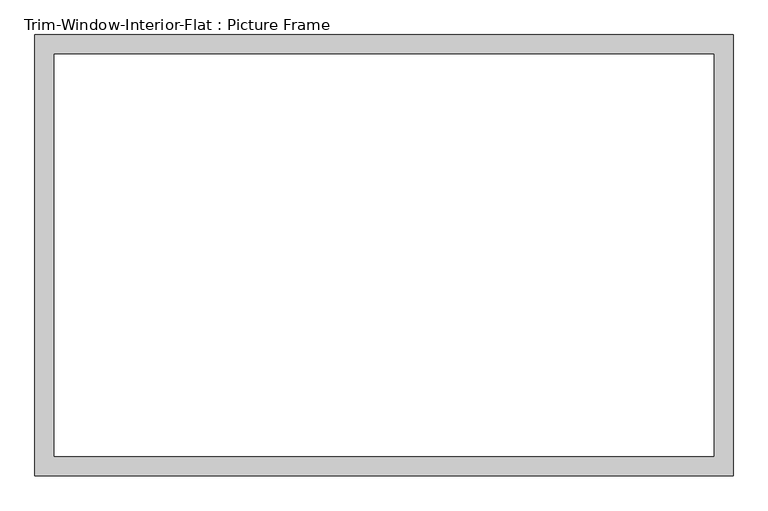
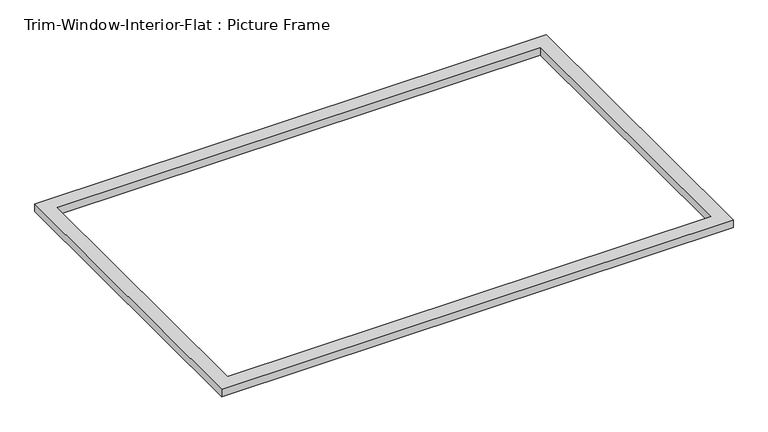
"""IFC4 building model written with IfcOpenShell, lengths in millimetres: proxy geometry, Trim-Window-Interior-Flat : Picture Frame."""

from ifc_helpers import new_model, si_unit, origin, origin_with_axes, place, context, project, spatial, polyline, outline, extrude, source, transform, mapped, element, save


def trim_window_interior_flat_picture_frame_b9d4c0b4(model_context):
    return source(origin(), model_context, "Body", "SweptSolid", [
        extrude(outline(polyline([(1035.05, 44.45), (1035.05, -1263.65), (-1035.05, -1263.65), (-1035.05, 44.45), (1035.05, 44.45)]), holes=[polyline([(977.9, -12.7), (-977.9, -12.7), (-977.9, -1206.5), (977.9, -1206.5), (977.9, -12.7)])]), origin_with_axes(), (0.0, 0.0, 1.0), 31.75),
    ])


if __name__ == "__main__":
    model = new_model("IFC4")
    model_context = context("Model", 3, world=origin())
    ifc_project = project(units=[si_unit("LENGTHUNIT", "METRE", prefix="MILLI")], contexts=[model_context])
    site = spatial("IfcSite", under=ifc_project)
    building = spatial("IfcBuilding", under=site)
    placement = place(None, origin())
    trim_window_interior_flat_picture_frame_shape = trim_window_interior_flat_picture_frame_b9d4c0b4(model_context)
    element("IfcBuildingElementProxy", 1, Name="Trim-Window-Interior-Flat : Picture Frame", ObjectType="Trim-Window-Interior-Flat : Picture Frame", at=placement, inside=building, context=model_context, shape_type="MappedRepresentation", body=[
        mapped(trim_window_interior_flat_picture_frame_shape, transform((0.0, 0.0, 0.0), x_axis=(1.0, 0.0, 0.0), y_axis=(0.0, 1.0, 0.0), z_axis=(0.0, 0.0, 1.0))),
    ])
    save(model, "model.ifc")

# Revit data of these elements
# Type "Trim-Window-Interior-Flat : Picture Frame"
#   Trim Thickness_Picture Frame = 0' - 1 1/4"
#   Trim Width = 0' - 2 1/4"
#   Trim Thickness_with Sill = 0' - 0 3/4"
#   Sill Thickness = 0' - 1 1/4"
#   Opening Width [instance default] = 2' - 0"
#   Opening Height [instance default] = 3' - 0"
#   Default Elevation = 4' - 0"
#   Sill = no
#   Picture Frame = yes
#   Trim Material [instance default] = none
# Element 1 (IfcBuildingElementProxy, "Trim-Window-Interior-Flat : Picture Frame")
#   Opening Width = 6' - 6"
#   Opening Height = 4' - 0"
#   Trim Material = Wood - Stained
#   Materials on its faces: "Wood - Stained"
# Materials
#   "Wood - Stained": class "Wood", colour RGB 224 178 126, transparency 0, Cost = 0
